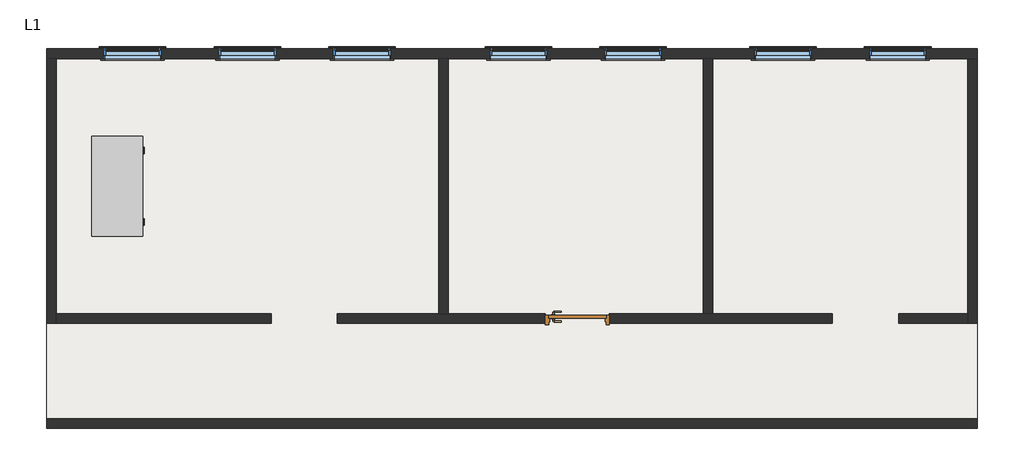
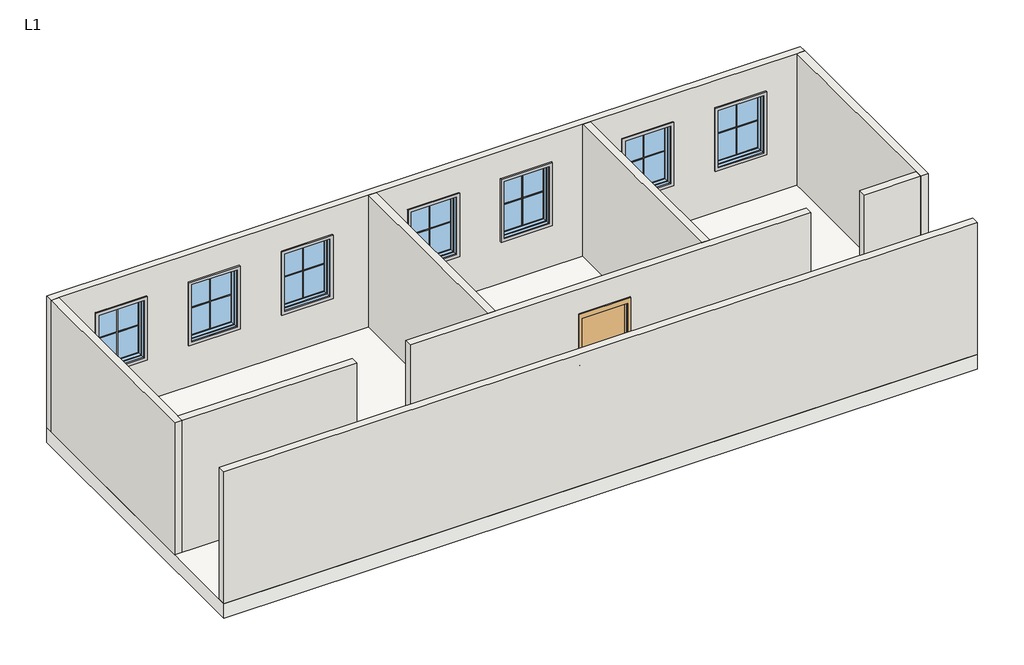
# One storey: 21 proxies, 9 walls, 7 windows, 1 door, 1 furniture element, 1 slab.
# Revit data of these elements (continued)
# Project information
#   Organization Name = "Organization Name"
#   Organization Description = "Organization Description"
#   Building Name = "Building Name"
#   Project Issue Date = "Issue Date"
#   Project Status = "Project Status"
#   Client Name = "Client Name"
#   Project Address = "Enter address here\nAddress Line 2"
#   Project Name = "Project Name"
#   Project Number = "Project Number"
# Type "M_Muntin Pattern_2x2 : M_Muntin Pattern_2x2"
#   Width [instance default] = 1200 mm
#   Thickness = 12.7 mm
#   Height [instance default] = 1200 mm
#   Distance = 19.05 mm
#   Interior Material [instance default] = none
#   Exterior Material [instance default] = none
#   Default Elevation = 0
# Type "M_Trim-Window-Exterior-Flat : with Sill"
#   Trim Width = 60 mm
#   Trim Thickness_Picture Frame = 30 mm
#   Trim Thickness_with Sill = 19.05 mm
#   Sill Thickness = 30 mm
#   Opening Width [instance default] = 600 mm
#   Opening Height [instance default] = 900 mm
#   Default Elevation = 1200 mm
#   Sill = yes
#   Picture Frame = no
#   Trim Material [instance default] = none
# Type "M_Trim-Window-Interior-Flat : Picture Frame"
#   Trim Thickness_Picture Frame = 30 mm
#   Trim Width = 60 mm
#   Trim Thickness_with Sill = 20 mm
#   Sill Thickness = 30 mm
#   Opening Width [instance default] = 600 mm
#   Opening Height [instance default] = 900 mm
#   Default Elevation = 1200 mm
#   Sill = no
#   Picture Frame = yes
#   Trim Material [instance default] = none
# Type "M_Door-Passage-Single-Flush : 900 x 2100mm"
#   Type Mark = "38"
#   Analytic Construction = "Wooden"
#   Thickness = 45 mm
#   Thermal Resistance (R) = 0.455703 (m²·K)/W
#   Swing Angle [instance default] = 90.00°
#   Strike Height = 1000 mm
#   Rough Width [instance default] = 1000 mm
#   Rough Height [instance default] = 2200 mm
#   MF Opening Height [instance default] = 100 mm
#   MF Opening Width [instance default] = 100 mm
#   Inset Calculate [instance default] = 105 mm
#   Masonry Inset [instance default] = 25 mm
#   Height = 2100 mm
#   Width = 900 mm
#   Heat Transfer Coefficient (U) = 2.19465 W/(m²·K)
#   Masonry Frame Depth = 150 mm
#   Masonry Frame [instance default] = yes
#   Function = 1
#   Dry Wall Frame [instance default] = no
#   Panel Material = Wood - Birch
#   Frame Material = Metal - Paint Finish - Grey
#   Door Handle Material = Aluminum
#   Visual Light Transmittance = 0
#   Solar Heat Gain Coefficient = 0
#   Wall Closure = (empty or 0)
# Type "M_Desk : 1525 x 762mm Student"
#   Depth = 762 mm
#   Height = 762 mm
#   Leg Height = 152 mm
#   Width = 1525 mm
#   Body Material = Laminate, Ivory, Matte
#   Handle/Leg Material = Steel, Chrome Plated
#   Top Material = Cherry
#   Default Elevation = 0
# Type "Generic 300mm"
#   Description = "Generic Floor (Material By Category), 300mm thick"
#   Function = 0
#   Layers, outside or top first: 300 mm no material (function 1)
# Type "Generic - 150mm"
#   Description = "Generic Wall (Material By Category), 150mm thick"
#   Type Mark = "G04"
#   Layers, outside or top first: 150 mm no material (function 1)
# Type "M_Window-Fixed : 900 x 1200mm"
#   Type Mark = "36"
#   Fire Rating = "0.5h"
#   Analytic Construction = "Double glazing - domestic"
#   Window Inset [instance default] = 0 mm
#   Wall Thickness [instance default] = 150 mm
#   Visual Light Transmittance = 0.81
#   Thermal Resistance (R) = 0.319569 (m²·K)/W
#   Solar Heat Gain Coefficient = 0.76
#   Rough Width = 915 mm
#   Rough Height = 1215 mm
#   Interior Wall Closure [instance default] = 54.75 mm
#   Height = 1200 mm
#   Heat Transfer Coefficient (U) = 3.12929 W/(m²·K)
#   Frame Extension [instance default] = 6.35 mm
#   Exterior Wall Closure [instance default] = 31.75 mm
#   Extension Jamb [instance default] = 54.75 mm
#   Default Sill Height = 900 mm
#   Width = 900 mm
#   Muntin Visibility = yes
#   Interior Trim Visibility [instance default] = yes
#   Exterior Trim Visibility [instance default] = yes
#   Extension Jamb Visibility [instance default] = yes
#   Muntin Pattern = M_Muntin Pattern_2x2 : M_Muntin Pattern_2x2
#   Interior Trim Material = Wood - Stained
#   Interior Trim = M_Trim-Window-Interior-Flat : Picture Frame
#   Interior Frame Material = Wood - Stained
#   Glass Panel Material = Glass
#   Exterior Trim Material = Clad - White
#   Exterior Trim = M_Trim-Window-Exterior-Flat : with Sill
#   Exterior Frame Material = Clad - White
#   Wall Closure = (empty or 0)
# Elements 1, 2, 3, 4, 5, 6, 7 (IfcBuildingElementProxy, "M_Muntin Pattern_2x2 : M_Muntin Pattern_2x2")
#   Width = 823.8 mm
#   Height = 1123.8 mm
#   Interior Material = Wood - Stained
#   Exterior Material = Clad - White
#   Phase Created = New Construction
#   Materials on its faces: "Clad - White", "Wood - Stained"
# Elements 8, 9, 10, 11, 12, 13, 14 (IfcBuildingElementProxy, "M_Trim-Window-Exterior-Flat : with Sill")
#   Opening Width = 900 mm
#   Opening Height = 1200 mm
#   Trim Material = Clad - White
#   Phase Created = New Construction
#   Materials on its faces: "Clad - White"
# Elements 15, 16, 17, 18, 19, 20, 21 (IfcBuildingElementProxy, "M_Trim-Window-Interior-Flat : Picture Frame")
#   Opening Width = 900 mm
#   Opening Height = 1200 mm
#   Trim Material = Wood - Stained
#   Phase Created = New Construction
#   Materials on its faces: "Wood - Stained"
# Element 22 (IfcDoor, "M_Door-Passage-Single-Flush : 900 x 2100mm")
#   Swing Angle = 90.00°
#   Rough Width = 1000 mm
#   Rough Height = 2200 mm
#   Masonry Inset = 25 mm
#   MF Opening Width = 100 mm
#   MF Opening Height = 100 mm
#   Inset Calculate = 105 mm
#   Masonry Frame = yes
#   Dry Wall Frame = no
#   Phase Created = New Construction
#   Materials on its faces: "Aluminum", "Metal - Paint Finish - Grey", "Wood - Birch"
# Element 23 (IfcFurniture, "M_Desk : 1525 x 762mm Student")
#   Phase Created = New Construction
#   Materials on its faces: "Steel, Chrome Plated", "Laminate, Ivory, Matte", "Cherry"
# Element 24 (IfcSlab, "Generic 300mm")
#   Height Offset From Level = 0 mm
#   Phase Created = New Construction
#   Materials on its faces: "Default Floor"
# Elements 25, 26, 27, 28, 29, 30, 31, 32, 33 (IfcWall, "Generic - 150mm")
#   Top Offset = 0 mm
#   Base Offset = 0 mm
#   Unconnected Height = 2700 mm
#   wall height = 2700 mm
#   Phase Created = New Construction
#   Base Constraint = L1
#   Materials on its faces: "Default Wall"
# Element 34 (IfcWindow, "M_Window-Fixed : 900 x 1200mm")
#   Mark = "100"
#   Window Inset = 0 mm
#   Interior Wall Closure = 54.75 mm
#   Frame Extension = 6.35 mm
#   Exterior Wall Closure = 31.75 mm
#   Interior Trim Visibility = yes
#   Exterior Trim Visibility = yes
#   Phase Created = New Construction
#   Materials on its faces: "Wood - Stained", "Glass", "Clad - White"
# Element 35 (IfcWindow, "M_Window-Fixed : 900 x 1200mm")
#   Mark = "101"
#   Window Inset = 0 mm
#   Interior Wall Closure = 54.75 mm
#   Frame Extension = 6.35 mm
#   Exterior Wall Closure = 31.75 mm
#   Interior Trim Visibility = yes
#   Exterior Trim Visibility = yes
#   Phase Created = New Construction
#   Materials on its faces: "Wood - Stained", "Glass", "Clad - White"
# Element 36 (IfcWindow, "M_Window-Fixed : 900 x 1200mm")
#   Mark = "102"
#   Window Inset = 0 mm
#   Interior Wall Closure = 54.75 mm
#   Frame Extension = 6.35 mm
#   Exterior Wall Closure = 31.75 mm
#   Interior Trim Visibility = yes
#   Exterior Trim Visibility = yes
#   Phase Created = New Construction
#   Materials on its faces: "Wood - Stained", "Glass", "Clad - White"
# Element 37 (IfcWindow, "M_Window-Fixed : 900 x 1200mm")
#   Mark = "103"
#   Window Inset = 0 mm
#   Interior Wall Closure = 54.75 mm
#   Frame Extension = 6.35 mm
#   Exterior Wall Closure = 31.75 mm
#   Interior Trim Visibility = yes
#   Exterior Trim Visibility = yes
#   Phase Created = New Construction
#   Materials on its faces: "Wood - Stained", "Glass", "Clad - White"
# Element 38 (IfcWindow, "M_Window-Fixed : 900 x 1200mm")
#   Mark = "104"
#   Window Inset = 0 mm
#   Interior Wall Closure = 54.75 mm
#   Frame Extension = 6.35 mm
#   Exterior Wall Closure = 31.75 mm
#   Interior Trim Visibility = yes
#   Exterior Trim Visibility = yes
#   Phase Created = New Construction
#   Materials on its faces: "Wood - Stained", "Glass", "Clad - White"
# Element 39 (IfcWindow, "M_Window-Fixed : 900 x 1200mm")
#   Mark = "105"
#   Window Inset = 0 mm
#   Interior Wall Closure = 54.75 mm
#   Frame Extension = 6.35 mm
#   Exterior Wall Closure = 31.75 mm
#   Interior Trim Visibility = yes
#   Exterior Trim Visibility = yes
#   Phase Created = New Construction
#   Materials on its faces: "Wood - Stained", "Glass", "Clad - White"
# Element 40 (IfcWindow, "M_Window-Fixed : 900 x 1200mm")
#   Mark = "106"
#   Window Inset = 0 mm
#   Interior Wall Closure = 54.75 mm
#   Frame Extension = 6.35 mm
#   Exterior Wall Closure = 31.75 mm
#   Interior Trim Visibility = yes
#   Exterior Trim Visibility = yes
#   Phase Created = New Construction
#   Materials on its faces: "Wood - Stained", "Glass", "Clad - White"
# Materials
#   "Wood - Birch": class "Wood", colour RGB 173 132 96, transparency 0, Cost = 0
#   "Metal - Paint Finish - Grey": class "Paint", colour RGB 178 178 178, transparency 0, Cost = 0
#   "Aluminum": class "Metal", colour RGB 244 245 246, transparency 0, Description = "Aluminum 6061", Cost = 0
#   "Laminate, Ivory, Matte": class "Plastic", colour RGB 244 244 244, transparency 0, Description = "Plastic Laminate - Ivory, Matte", Cost = 0
#   "Steel, Chrome Plated": class "Metal", colour RGB 17 17 17, transparency 0, Description = "Chromiuim plated steel", Cost = 0
#   "Cherry": class "Wood", colour RGB 158 77 40, transparency 0, Description = "Prunus Serotina", Cost = 0
#   "Wood - Stained": class "Wood", colour RGB 173 132 96, transparency 0, Cost = 0
#   "Glass": class "Glass", colour RGB 245 245 243, transparency 1, Description = "Soda Lime Glass", Cost = 0
#   "Clad - White": class "Wood", colour RGB 245 245 243, transparency 0, Cost = 0
#   "Default Floor": class "Miscellaneous", colour RGB 128 128 128, transparency 0, Cost = 0
#   "Default Wall": class "Miscellaneous", colour RGB 192 192 192, transparency 0, Cost = 0
